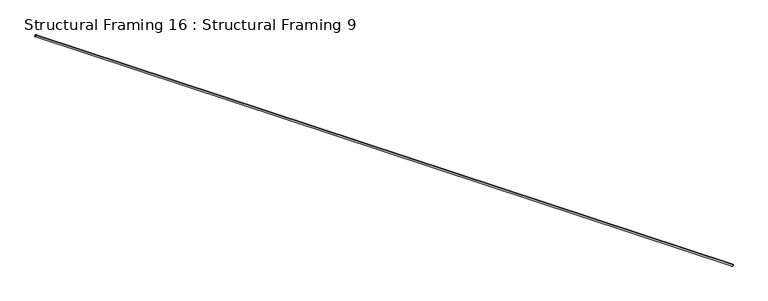
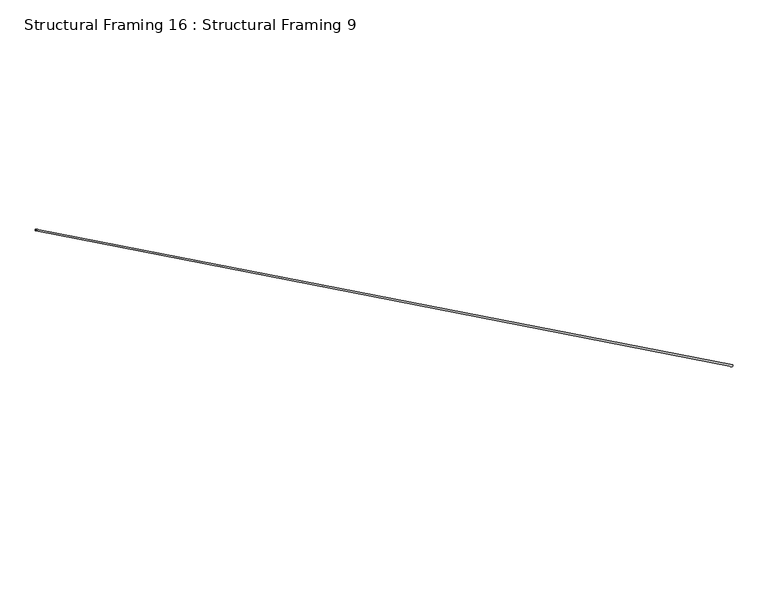
"""IFC4 building model written with IfcOpenShell, lengths in millimetres: beam geometry, Structural Framing 16 : Structural Framing 9."""

from ifc_helpers import new_model, si_unit, point, frame, origin, origin_2d, place, context, project, spatial, circle_curve, trimmed, segment, composite_curve, outline, extrude, source, transform, mapped, element, save


def structural_framing_16_structural_framing_9_c8541427(model_context):
    return source(origin(), model_context, "Body", "SweptSolid", [
        extrude(outline(composite_curve([segment(trimmed(circle_curve(origin_2d(), 6.35), [point((0.0, 6.35))], [point((0.0, -6.3499999))], False, "CARTESIAN"), True, "CONTINUOUS"), segment(trimmed(circle_curve(origin_2d(), 6.35), [point((0.0, -6.3499999))], [point((0.0, 6.35))], False, "CARTESIAN"), True, "CONTINUOUS")], self_intersect=False)), frame((28306.0390052, 2544.1506464, 2962.9722581), z_axis=(-0.8890536510975655, 0.29307835176728264, 0.3516940221207373), x_axis=(0.0, 0.7682212795973775, -0.640184399664478)), (0.0, 0.0, 1.0), 5574.8064179),
    ])


if __name__ == "__main__":
    model = new_model("IFC4")
    model_context = context("Model", 3, world=origin())
    ifc_project = project(units=[si_unit("LENGTHUNIT", "METRE", prefix="MILLI")], contexts=[model_context])
    site = spatial("IfcSite", under=ifc_project)
    building = spatial("IfcBuilding", under=site)
    placement = place(None, origin())
    structural_framing_16_structural_framing_9_shape = structural_framing_16_structural_framing_9_c8541427(model_context)
    element("IfcBeam", 1, ObjectType="Structural Framing 16 : Structural Framing 9", at=placement, inside=building, context=model_context, shape_type="MappedRepresentation", body=[
        mapped(structural_framing_16_structural_framing_9_shape, transform((0.0, 0.0, 0.0), x_axis=(1.0, 0.0, 0.0), y_axis=(0.0, 1.0, 0.0), z_axis=(0.0, 0.0, 1.0))),
    ])
    save(model, "model.ifc")

# Revit data of these elements
# Type "Structural Framing 16 : Structural Framing 9"
#   Structural Material [instance default] = EXISTING LATERAL BRACING (1/4" CABLE)
# Element 1 (IfcBeam, "Structural Framing 16 : Structural Framing 9")
#   Materials on its faces: "EXISTING LATERAL BRACING (1/4\" CABLE)"
# Materials
#   "EXISTING LATERAL BRACING (1/4\" CABLE)": class "Generic", colour RGB 120 120 120, transparency 0, Cost = 0
